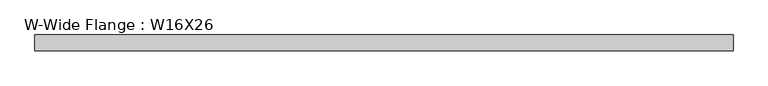
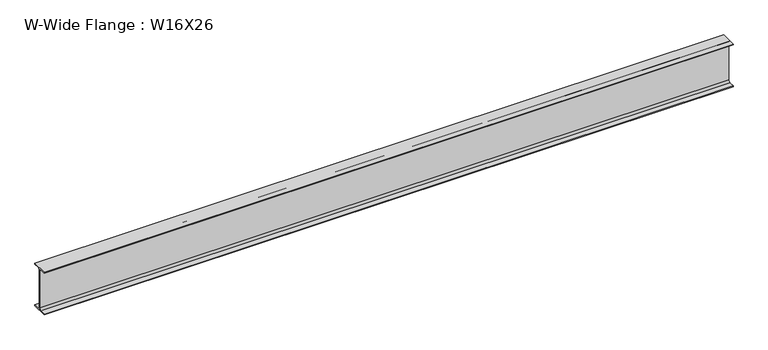
"""IFC4 building model written with IfcOpenShell, lengths in millimetres: beam geometry, W-Wide Flange : W16X26."""

import ifcopenshell
import ifcopenshell.guid

model = None  # the IFC model being written
_history = None  # IfcOwnerHistory: only IFC2X3 demands one
_inside = {}  # id of a spatial element -> (the spatial element, [elements in it])
_under = {}  # id of a project, library or spatial element -> (it, [spatial elements below it])
_declared = {}  # id of a project -> (the project, [libraries it declares])
_typed = {}  # id of a type object -> (the type object, [elements of that type])
_made_of = {}  # id of a material, layer set ... -> (it, [elements and type objects made of it])


def new_model(schema):
    """Start an empty IFC model of exactly this schema.

    Asked for "IFC4X3", IfcOpenShell would pick the latest addendum, in which some entities
    have other attributes; the version numbers below select the first issue.
    IFC2X3 requires an IfcOwnerHistory on every rooted entity: one is made here for all.
    """
    global model, _history
    if schema == "IFC4X3":
        model = ifcopenshell.file(schema_version=(4, 3, 0, 0))
    else:
        model = ifcopenshell.file(schema=schema)
    _inside.clear()
    _under.clear()
    _declared.clear()
    _typed.clear()
    _made_of.clear()
    _history = None
    if model.schema == "IFC2X3":
        org = make("IfcOrganization", Name="unknown")
        user = make(
            "IfcPersonAndOrganization",
            ThePerson=make("IfcPerson", FamilyName="unknown"),
            TheOrganization=org,
        )
        app = make(
            "IfcApplication",
            ApplicationDeveloper=org,
            Version="unknown",
            ApplicationFullName="unknown",
            ApplicationIdentifier="unknown",
        )
        _history = make(
            "IfcOwnerHistory",
            OwningUser=user,
            OwningApplication=app,
            ChangeAction="ADDED",
            CreationDate=0,
        )
    return model


def make(cls, **values):
    """One entity of the class cls with the attributes given. An attribute that is None is left unset."""
    return model.create_entity(
        cls, **{name: value for name, value in values.items() if value is not None}
    )


def rooted(cls, **values):
    """An entity with a GlobalId (a new one), such as an element, a storey or a relation."""
    return make(cls, GlobalId=ifcopenshell.guid.new(), OwnerHistory=_history, **values)


def si_unit(unit_type, name, prefix=None):
    """IfcSIUnit, for example si_unit("LENGTHUNIT", "METRE", prefix="MILLI")."""
    return make("IfcSIUnit", UnitType=unit_type, Prefix=prefix, Name=name)


def assignment(units):
    """IfcUnitAssignment: the units of a project."""
    return None if units is None else make("IfcUnitAssignment", Units=units)


def point(xyz):
    """IfcCartesianPoint."""
    return None if xyz is None else make("IfcCartesianPoint", Coordinates=xyz)


def direction(xyz):
    """IfcDirection."""
    return None if xyz is None else make("IfcDirection", DirectionRatios=xyz)


def frame(location, z_axis=None, x_axis=None):
    """IfcAxis2Placement3D, a coordinate frame: its origin and axes. An axis left out is left unset."""
    return make(
        "IfcAxis2Placement3D",
        Location=point(location),
        Axis=direction(z_axis),
        RefDirection=direction(x_axis),
    )


def frame_2d(location, x_axis=None):
    """IfcAxis2Placement2D, a coordinate frame in the plane: its origin and x axis."""
    return make(
        "IfcAxis2Placement2D", Location=point(location), RefDirection=direction(x_axis)
    )


def origin():
    """The frame at (0, 0, 0) with its axes left unset."""
    return frame((0.0, 0.0, 0.0))


def place(relative_to, where):
    """IfcLocalPlacement: puts the frame where relative to a parent placement (None: the world)."""
    return make(
        "IfcLocalPlacement", PlacementRelTo=relative_to, RelativePlacement=where
    )


def context(
    kind, dimensions, precision=None, world=None, true_north=None, identifier=None
):
    """IfcGeometricRepresentationContext, for example the 3D "Model" context."""
    return make(
        "IfcGeometricRepresentationContext",
        ContextIdentifier=identifier,
        ContextType=kind,
        CoordinateSpaceDimension=dimensions,
        Precision=precision,
        WorldCoordinateSystem=world,
        TrueNorth=true_north,
    )


def project(units=None, contexts=None):
    """IfcProject with its units and contexts."""
    return rooted(
        "IfcProject",
        Name="project",
        RepresentationContexts=contexts,
        UnitsInContext=assignment(units),
    )


def spatial(cls, under=None, at=None, **own):
    """A site, building, storey or space (cls), placed at a placement, below another one or the project."""
    s = rooted(cls, ObjectPlacement=at, **own)
    if under is not None:
        _under.setdefault(under.id(), (under, []))[1].append(s)
    return s


def polyline(points):
    """IfcPolyline through the points."""
    return make("IfcPolyline", Points=[point(p) for p in points])


def circle_curve(where, radius):
    """IfcCircle in the frame where."""
    return make("IfcCircle", Position=where, Radius=radius)


def trimmed(basis, trim1, trim2, sense, master):
    """IfcTrimmedCurve: the piece of a basis curve between two trims."""
    return make(
        "IfcTrimmedCurve",
        BasisCurve=basis,
        Trim1=trim1,
        Trim2=trim2,
        SenseAgreement=sense,
        MasterRepresentation=master,
    )


def segment(curve, same_sense, transition):
    """IfcCompositeCurveSegment."""
    return make(
        "IfcCompositeCurveSegment",
        Transition=transition,
        SameSense=same_sense,
        ParentCurve=curve,
    )


def composite_curve(segments, self_intersect=None):
    """IfcCompositeCurve: segments joined end to end."""
    return make("IfcCompositeCurve", Segments=segments, SelfIntersect=self_intersect)


def outline(outer, holes=None, kind="AREA"):
    """IfcArbitraryClosedProfileDef: a profile drawn as a closed curve; with holes, ...WithVoids."""
    if holes is None:
        return make("IfcArbitraryClosedProfileDef", ProfileType=kind, OuterCurve=outer)
    return make(
        "IfcArbitraryProfileDefWithVoids",
        ProfileType=kind,
        OuterCurve=outer,
        InnerCurves=holes,
    )


def extrude(swept, where, along, depth):
    """IfcExtrudedAreaSolid: the profile swept, set in the frame where, extruded along a direction by depth."""
    return make(
        "IfcExtrudedAreaSolid",
        SweptArea=swept,
        Position=where,
        ExtrudedDirection=direction(along),
        Depth=depth,
    )


def shape(context_of_items, identifier, shape_type, items):
    """IfcShapeRepresentation: the items that make up one representation, for example the "Body"."""
    return make(
        "IfcShapeRepresentation",
        ContextOfItems=context_of_items,
        RepresentationIdentifier=identifier,
        RepresentationType=shape_type,
        Items=items,
    )


def source(mapping_origin, context_of_items, identifier, shape_type, items):
    """IfcRepresentationMap: a shape defined once, which mapped items show again and again."""
    return make(
        "IfcRepresentationMap",
        MappingOrigin=mapping_origin,
        MappedRepresentation=shape(context_of_items, identifier, shape_type, items),
    )


def transform(
    local_origin,
    x_axis=None,
    y_axis=None,
    z_axis=None,
    scale=None,
    scale2=None,
    scale3=None,
    uniform=True,
):
    """IfcCartesianTransformationOperator3D, or its non-uniform kind. x_axis, y_axis, z_axis: its Axis1, 2, 3."""
    if uniform:
        return make(
            "IfcCartesianTransformationOperator3D",
            Axis1=direction(x_axis),
            Axis2=direction(y_axis),
            LocalOrigin=point(local_origin),
            Scale=scale,
            Axis3=direction(z_axis),
        )
    return make(
        "IfcCartesianTransformationOperator3DnonUniform",
        Axis1=direction(x_axis),
        Axis2=direction(y_axis),
        LocalOrigin=point(local_origin),
        Scale=scale,
        Axis3=direction(z_axis),
        Scale2=scale2,
        Scale3=scale3,
    )


def mapped(mapping_source, mapping_target):
    """IfcMappedItem: shows the shape of a source again, moved by a transform."""
    return make(
        "IfcMappedItem", MappingSource=mapping_source, MappingTarget=mapping_target
    )


def made_of(thing, what):
    """Note that an element or type object is made of a material, layer set ...; save() writes the relation."""
    if what is not None:
        _made_of.setdefault(what.id(), (what, []))[1].append(thing)
    return thing


def element(
    cls,
    number,
    at=None,
    inside=None,
    cuts=None,
    type_object=None,
    material=None,
    context=None,
    identifier="Body",
    shape_type=None,
    held_by="IfcProductDefinitionShape",
    body=None,
    shapes=None,
    **own,
):
    """One element of the class cls, such as IfcWall. Its Tag is "e" and its number.

    at: its placement. inside: the storey or other place that contains it. cuts: it is an
    opening in that element (IfcRelVoidsElement). A single representation is given by context,
    identifier, shape_type and body (its items); several are given by shapes. held_by: the class
    of the entity that holds the representations. save() writes the other relations.
    """
    e = rooted(cls, Tag="e%d" % number, ObjectPlacement=at, **own)
    if body is not None:
        shapes = [shape(context, identifier, shape_type, body)]
    if shapes is not None:
        e.Representation = make(held_by, Representations=shapes)
    if inside is not None:
        _inside.setdefault(inside.id(), (inside, []))[1].append(e)
    if cuts is not None:
        rooted(
            "IfcRelVoidsElement", RelatingBuildingElement=cuts, RelatedOpeningElement=e
        )
    if type_object is not None:
        _typed.setdefault(type_object.id(), (type_object, []))[1].append(e)
    return made_of(e, material)


def aggregate(whole, parts):
    """IfcRelAggregates: a whole, such as a stair, and the parts it consists of."""
    return rooted("IfcRelAggregates", RelatingObject=whole, RelatedObjects=parts)


def save(model, path):
    """Write the relations noted so far, then the file.

    IfcRelAggregates (storeys below a building ...), IfcRelContainedInSpatialStructure (elements
    in a storey), IfcRelDefinesByType, IfcRelAssociatesMaterial and IfcRelDeclares: one each for
    every whole, place, type object, material and project.
    """
    for whole, parts in _under.values():
        aggregate(whole, parts)
    for where, things in _inside.values():
        rooted(
            "IfcRelContainedInSpatialStructure",
            RelatedElements=things,
            RelatingStructure=where,
        )
    for kind, things in _typed.values():
        rooted("IfcRelDefinesByType", RelatedObjects=things, RelatingType=kind)
    for what, things in _made_of.values():
        rooted("IfcRelAssociatesMaterial", RelatedObjects=things, RelatingMaterial=what)
    for by, libraries in _declared.values():
        rooted("IfcRelDeclares", RelatingContext=by, RelatedDefinitions=libraries)
    model.write(path)


def w_wide_flange_w16x26_6f425e70(model_context):
    return source(origin(), model_context, "Body", "SweptSolid", [
        extrude(outline(composite_curve([segment(polyline([(69.85, -190.627), (69.85, -199.39), (-69.85, -199.39), (-69.85, -190.627), (-21.3995, -190.627)]), True, "CONTINUOUS"), segment(trimmed(circle_curve(frame_2d((-21.3995, -172.4025)), 18.2245), [point((-21.3995, -190.627))], [point((-3.175, -172.4025))], True, "CARTESIAN"), True, "CONTINUOUS"), segment(polyline([(-3.175, -172.4025), (-3.175, 172.4025)]), True, "CONTINUOUS"), segment(trimmed(circle_curve(frame_2d((-21.3995, 172.4025)), 18.2245), [point((-3.175, 172.4025))], [point((-21.3995, 190.627))], True, "CARTESIAN"), True, "CONTINUOUS"), segment(polyline([(-21.3995, 190.627), (-69.85, 190.627), (-69.85, 199.39), (69.85, 199.39), (69.85, 190.627), (21.3995, 190.627)]), True, "CONTINUOUS"), segment(trimmed(circle_curve(frame_2d((21.3995, 172.4025)), 18.2245), [point((21.3995, 190.627))], [point((3.175, 172.4025))], True, "CARTESIAN"), True, "CONTINUOUS"), segment(polyline([(3.175, 172.4025), (3.175, -172.4025)]), True, "CONTINUOUS"), segment(trimmed(circle_curve(frame_2d((21.3995, -172.4025)), 18.2245), [point((3.175, -172.4025))], [point((21.3995, -190.627))], True, "CARTESIAN"), True, "CONTINUOUS"), segment(polyline([(21.3995, -190.627), (69.85, -190.627)]), True, "CONTINUOUS")], self_intersect=False)), frame((-3035.3, 0.0, 0.0), z_axis=(1.0, 0.0, 0.0), x_axis=(0.0, 1.0, 0.0)), (0.0, 0.0, 1.0), 6070.6),
    ])


if __name__ == "__main__":
    model = new_model("IFC4")
    model_context = context("Model", 3, world=origin())
    ifc_project = project(units=[si_unit("LENGTHUNIT", "METRE", prefix="MILLI")], contexts=[model_context])
    site = spatial("IfcSite", under=ifc_project)
    building = spatial("IfcBuilding", under=site)
    placement = place(None, origin())
    w_wide_flange_w16x26_shape = w_wide_flange_w16x26_6f425e70(model_context)
    element("IfcBeam", 1, ObjectType="W-Wide Flange : W16X26", at=placement, inside=building, context=model_context, shape_type="MappedRepresentation", body=[
        mapped(w_wide_flange_w16x26_shape, transform((0.0, 0.0, 0.0), x_axis=(1.0, 0.0, 0.0), y_axis=(0.0, 1.0, 0.0), z_axis=(0.0, 0.0, 1.0))),
    ])
    save(model, "model.ifc")

# Revit data of these elements
# Type "W-Wide Flange : W16X26"
#   Assembly Code = "B10"
#   W = 26
#   Length [instance default] = 5' - 0"
#   bf = 0' - 5 1/2"
#   d = 1' - 3.7"
#   k = 0' - 1 1/16"
#   k2 = 0' - 0.7175"
#   tf = 0' - 0.345"
#   tw = 0' - 0 1/4"
#   A = 0.0533333 SF
#   Structural Material [instance default] = Steel ASTM A992
# Element 1 (IfcBeam, "W-Wide Flange : W16X26")
#   Materials on its faces: "Steel ASTM A992"
# Materials
#   "Steel ASTM A992": class "Metal", colour RGB 199 199 199, transparency 0, Description = "Structural steel 50ksi", Cost = 0
